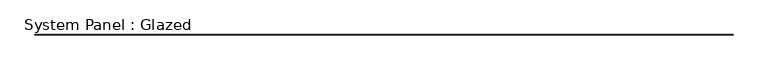
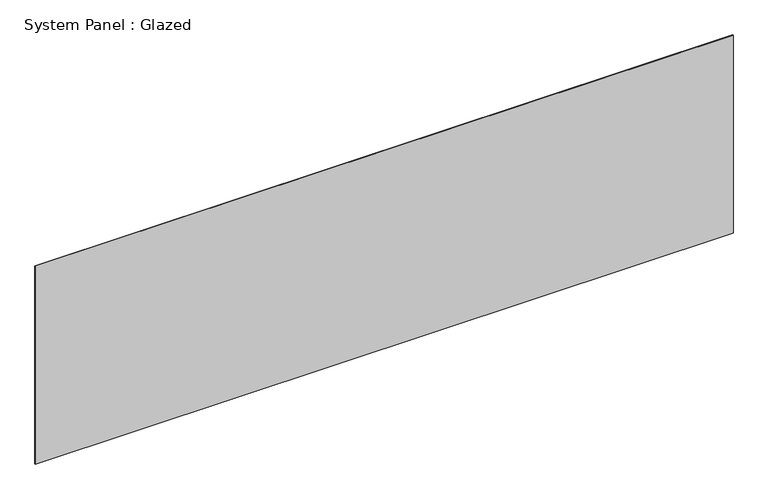
"""IFC4 building model written with IfcOpenShell, lengths in millimetres: plate geometry, System Panel : Glazed."""

from ifc_helpers import new_model, si_unit, origin, origin_with_axes, place, context, project, spatial, polyline, outline, extrude, source, transform, mapped, element, save


def system_panel_glazed_15d59c4f(model_context):
    return source(origin(), model_context, "Body", "SweptSolid", [
        extrude(outline(polyline([(14987.75, 24.5), (-14987.75, 24.5), (-14987.75, 49.5), (14987.75, 49.5), (14987.75, 24.5)])), origin_with_axes(), (0.0, 0.0, 1.0), 9000.0),
    ])


if __name__ == "__main__":
    model = new_model("IFC4")
    model_context = context("Model", 3, world=origin())
    ifc_project = project(units=[si_unit("LENGTHUNIT", "METRE", prefix="MILLI")], contexts=[model_context])
    site = spatial("IfcSite", under=ifc_project)
    building = spatial("IfcBuilding", under=site)
    placement = place(None, origin())
    system_panel_glazed_shape = system_panel_glazed_15d59c4f(model_context)
    element("IfcPlate", 1, ObjectType="System Panel : Glazed", at=placement, inside=building, context=model_context, shape_type="MappedRepresentation", body=[
        mapped(system_panel_glazed_shape, transform((0.0, 0.0, 0.0), x_axis=(1.0, 0.0, 0.0), y_axis=(0.0, 1.0, 0.0), z_axis=(0.0, 0.0, 1.0))),
    ])
    save(model, "model.ifc")

# Revit data of these elements
# Element 1 (IfcPlate, "System Panel : Glazed")
#   Materials on its faces: "Glass"
# Materials
#   "Glass": class "Glass", colour RGB 0 128 192, transparency 0.9
